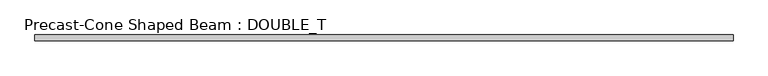
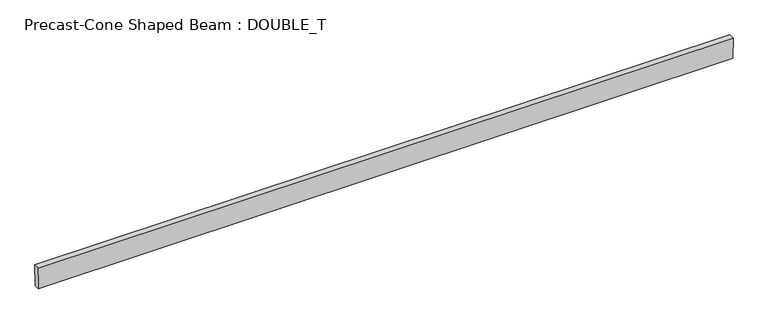
"""IFC4 building model written with IfcOpenShell, lengths in millimetres: beam geometry, Precast-Cone Shaped Beam : DOUBLE_T."""

from ifc_helpers import new_model, si_unit, frame, origin, place, context, project, spatial, polyline, outline, extrude, source, transform, mapped, element, save


def precast_cone_shaped_beam_double_t_5f2c7775(model_context):
    return source(origin(), model_context, "Body", "SweptSolid", [
        extrude(outline(polyline([(50.8, -228.6), (-50.8, -228.6), (-63.5, 228.6), (63.5, 228.6), (50.8, -228.6)])), frame((-7353.3, 0.0, 0.0), z_axis=(1.0, 0.0, 0.0), x_axis=(0.0, 1.0, 0.0)), (0.0, 0.0, 1.0), 14693.9),
    ])


if __name__ == "__main__":
    model = new_model("IFC4")
    model_context = context("Model", 3, world=origin())
    ifc_project = project(units=[si_unit("LENGTHUNIT", "METRE", prefix="MILLI")], contexts=[model_context])
    site = spatial("IfcSite", under=ifc_project)
    building = spatial("IfcBuilding", under=site)
    placement = place(None, origin())
    precast_cone_shaped_beam_double_t_shape = precast_cone_shaped_beam_double_t_5f2c7775(model_context)
    element("IfcBeam", 1, ObjectType="Precast-Cone Shaped Beam : DOUBLE_T", at=placement, inside=building, context=model_context, shape_type="MappedRepresentation", body=[
        mapped(precast_cone_shaped_beam_double_t_shape, transform((0.0, 0.0, 0.0), x_axis=(1.0, 0.0, 0.0), y_axis=(0.0, 1.0, 0.0), z_axis=(0.0, 0.0, 1.0))),
    ])
    save(model, "model.ifc")

# Revit data of these elements
# Type "Precast-Cone Shaped Beam : DOUBLE_T"
#   Top Width = 0' - 5"
#   Tie Rod Weight [instance default] = 30
#   Tie Rod W [instance default] = 0.0660938 kip
#   Single Rebar Weight [instance default] = 50
#   Single Rebar W [instance default] = 0.110156 kip
#   Rebar Grids Weight [instance default] = 100
#   Rebar Grids W [instance default] = 0.220313 kip
#   Depth = 1' - 6"
#   Bottom Width = 0' - 4"
#   Length [instance default] = 5' - 0"
#   Structural Material [instance default] = Concrete, Precast
#   Assembly Code = ""
# Element 1 (IfcBeam, "Precast-Cone Shaped Beam : DOUBLE_T")
#   Length = 49' - 3"
#   Structural Material = Concrete - Precast Concrete - Normal Weight Concrete - 5 ksi
#   Materials on its faces: "Concrete - Precast Concrete - Normal Weight Concrete - 5 ksi"
# Materials
#   "Concrete, Precast": class "Concrete", colour RGB 198 187 187, transparency 0, Description = "Precast concrete", Cost = 0
#   "Concrete - Precast Concrete - Normal Weight Concrete - 5 ksi": class "Concrete", colour RGB 198 187 187, transparency 0, Cost = 0
